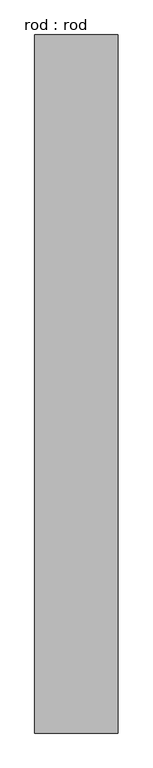
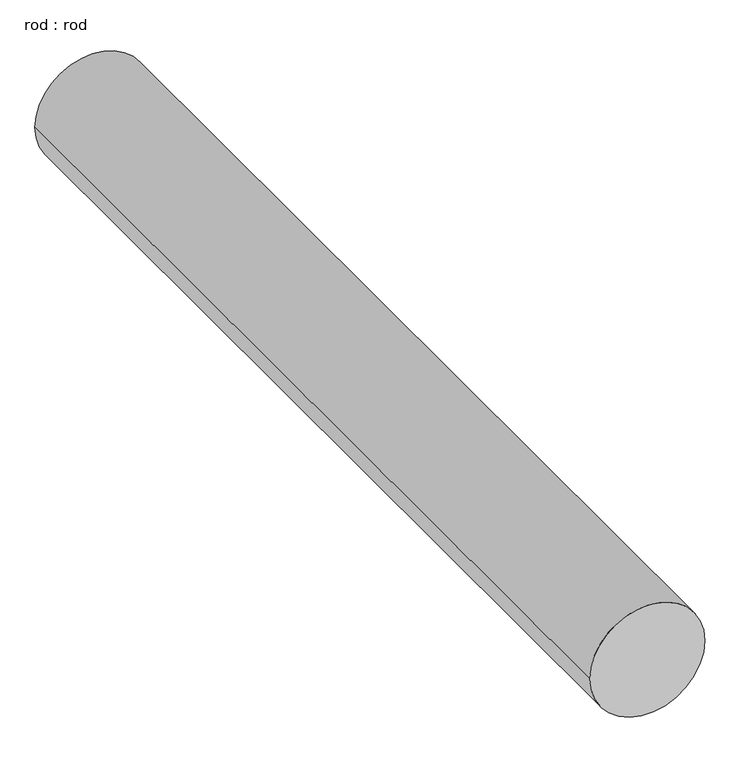
"""IFC4 building model written with IfcOpenShell, lengths in millimetres: proxy geometry, rod : rod."""

import ifcopenshell
import ifcopenshell.guid

model = None  # the IFC model being written
_history = None  # IfcOwnerHistory: only IFC2X3 demands one
_inside = {}  # id of a spatial element -> (the spatial element, [elements in it])
_under = {}  # id of a project, library or spatial element -> (it, [spatial elements below it])
_declared = {}  # id of a project -> (the project, [libraries it declares])
_typed = {}  # id of a type object -> (the type object, [elements of that type])
_made_of = {}  # id of a material, layer set ... -> (it, [elements and type objects made of it])


def new_model(schema):
    """Start an empty IFC model of exactly this schema.

    Asked for "IFC4X3", IfcOpenShell would pick the latest addendum, in which some entities
    have other attributes; the version numbers below select the first issue.
    IFC2X3 requires an IfcOwnerHistory on every rooted entity: one is made here for all.
    """
    global model, _history
    if schema == "IFC4X3":
        model = ifcopenshell.file(schema_version=(4, 3, 0, 0))
    else:
        model = ifcopenshell.file(schema=schema)
    _inside.clear()
    _under.clear()
    _declared.clear()
    _typed.clear()
    _made_of.clear()
    _history = None
    if model.schema == "IFC2X3":
        org = make("IfcOrganization", Name="unknown")
        user = make(
            "IfcPersonAndOrganization",
            ThePerson=make("IfcPerson", FamilyName="unknown"),
            TheOrganization=org,
        )
        app = make(
            "IfcApplication",
            ApplicationDeveloper=org,
            Version="unknown",
            ApplicationFullName="unknown",
            ApplicationIdentifier="unknown",
        )
        _history = make(
            "IfcOwnerHistory",
            OwningUser=user,
            OwningApplication=app,
            ChangeAction="ADDED",
            CreationDate=0,
        )
    return model


def make(cls, **values):
    """One entity of the class cls with the attributes given. An attribute that is None is left unset."""
    return model.create_entity(
        cls, **{name: value for name, value in values.items() if value is not None}
    )


def rooted(cls, **values):
    """An entity with a GlobalId (a new one), such as an element, a storey or a relation."""
    return make(cls, GlobalId=ifcopenshell.guid.new(), OwnerHistory=_history, **values)


def si_unit(unit_type, name, prefix=None):
    """IfcSIUnit, for example si_unit("LENGTHUNIT", "METRE", prefix="MILLI")."""
    return make("IfcSIUnit", UnitType=unit_type, Prefix=prefix, Name=name)


def assignment(units):
    """IfcUnitAssignment: the units of a project."""
    return None if units is None else make("IfcUnitAssignment", Units=units)


def point(xyz):
    """IfcCartesianPoint."""
    return None if xyz is None else make("IfcCartesianPoint", Coordinates=xyz)


def direction(xyz):
    """IfcDirection."""
    return None if xyz is None else make("IfcDirection", DirectionRatios=xyz)


def frame(location, z_axis=None, x_axis=None):
    """IfcAxis2Placement3D, a coordinate frame: its origin and axes. An axis left out is left unset."""
    return make(
        "IfcAxis2Placement3D",
        Location=point(location),
        Axis=direction(z_axis),
        RefDirection=direction(x_axis),
    )


def frame_2d(location, x_axis=None):
    """IfcAxis2Placement2D, a coordinate frame in the plane: its origin and x axis."""
    return make(
        "IfcAxis2Placement2D", Location=point(location), RefDirection=direction(x_axis)
    )


def origin():
    """The frame at (0, 0, 0) with its axes left unset."""
    return frame((0.0, 0.0, 0.0))


def place(relative_to, where):
    """IfcLocalPlacement: puts the frame where relative to a parent placement (None: the world)."""
    return make(
        "IfcLocalPlacement", PlacementRelTo=relative_to, RelativePlacement=where
    )


def context(
    kind, dimensions, precision=None, world=None, true_north=None, identifier=None
):
    """IfcGeometricRepresentationContext, for example the 3D "Model" context."""
    return make(
        "IfcGeometricRepresentationContext",
        ContextIdentifier=identifier,
        ContextType=kind,
        CoordinateSpaceDimension=dimensions,
        Precision=precision,
        WorldCoordinateSystem=world,
        TrueNorth=true_north,
    )


def project(units=None, contexts=None):
    """IfcProject with its units and contexts."""
    return rooted(
        "IfcProject",
        Name="project",
        RepresentationContexts=contexts,
        UnitsInContext=assignment(units),
    )


def spatial(cls, under=None, at=None, **own):
    """A site, building, storey or space (cls), placed at a placement, below another one or the project."""
    s = rooted(cls, ObjectPlacement=at, **own)
    if under is not None:
        _under.setdefault(under.id(), (under, []))[1].append(s)
    return s


def circle_curve(where, radius):
    """IfcCircle in the frame where."""
    return make("IfcCircle", Position=where, Radius=radius)


def trimmed(basis, trim1, trim2, sense, master):
    """IfcTrimmedCurve: the piece of a basis curve between two trims."""
    return make(
        "IfcTrimmedCurve",
        BasisCurve=basis,
        Trim1=trim1,
        Trim2=trim2,
        SenseAgreement=sense,
        MasterRepresentation=master,
    )


def segment(curve, same_sense, transition):
    """IfcCompositeCurveSegment."""
    return make(
        "IfcCompositeCurveSegment",
        Transition=transition,
        SameSense=same_sense,
        ParentCurve=curve,
    )


def composite_curve(segments, self_intersect=None):
    """IfcCompositeCurve: segments joined end to end."""
    return make("IfcCompositeCurve", Segments=segments, SelfIntersect=self_intersect)


def outline(outer, holes=None, kind="AREA"):
    """IfcArbitraryClosedProfileDef: a profile drawn as a closed curve; with holes, ...WithVoids."""
    if holes is None:
        return make("IfcArbitraryClosedProfileDef", ProfileType=kind, OuterCurve=outer)
    return make(
        "IfcArbitraryProfileDefWithVoids",
        ProfileType=kind,
        OuterCurve=outer,
        InnerCurves=holes,
    )


def extrude(swept, where, along, depth):
    """IfcExtrudedAreaSolid: the profile swept, set in the frame where, extruded along a direction by depth."""
    return make(
        "IfcExtrudedAreaSolid",
        SweptArea=swept,
        Position=where,
        ExtrudedDirection=direction(along),
        Depth=depth,
    )


def shape(context_of_items, identifier, shape_type, items):
    """IfcShapeRepresentation: the items that make up one representation, for example the "Body"."""
    return make(
        "IfcShapeRepresentation",
        ContextOfItems=context_of_items,
        RepresentationIdentifier=identifier,
        RepresentationType=shape_type,
        Items=items,
    )


def source(mapping_origin, context_of_items, identifier, shape_type, items):
    """IfcRepresentationMap: a shape defined once, which mapped items show again and again."""
    return make(
        "IfcRepresentationMap",
        MappingOrigin=mapping_origin,
        MappedRepresentation=shape(context_of_items, identifier, shape_type, items),
    )


def transform(
    local_origin,
    x_axis=None,
    y_axis=None,
    z_axis=None,
    scale=None,
    scale2=None,
    scale3=None,
    uniform=True,
):
    """IfcCartesianTransformationOperator3D, or its non-uniform kind. x_axis, y_axis, z_axis: its Axis1, 2, 3."""
    if uniform:
        return make(
            "IfcCartesianTransformationOperator3D",
            Axis1=direction(x_axis),
            Axis2=direction(y_axis),
            LocalOrigin=point(local_origin),
            Scale=scale,
            Axis3=direction(z_axis),
        )
    return make(
        "IfcCartesianTransformationOperator3DnonUniform",
        Axis1=direction(x_axis),
        Axis2=direction(y_axis),
        LocalOrigin=point(local_origin),
        Scale=scale,
        Axis3=direction(z_axis),
        Scale2=scale2,
        Scale3=scale3,
    )


def mapped(mapping_source, mapping_target):
    """IfcMappedItem: shows the shape of a source again, moved by a transform."""
    return make(
        "IfcMappedItem", MappingSource=mapping_source, MappingTarget=mapping_target
    )


def made_of(thing, what):
    """Note that an element or type object is made of a material, layer set ...; save() writes the relation."""
    if what is not None:
        _made_of.setdefault(what.id(), (what, []))[1].append(thing)
    return thing


def element(
    cls,
    number,
    at=None,
    inside=None,
    cuts=None,
    type_object=None,
    material=None,
    context=None,
    identifier="Body",
    shape_type=None,
    held_by="IfcProductDefinitionShape",
    body=None,
    shapes=None,
    **own,
):
    """One element of the class cls, such as IfcWall. Its Tag is "e" and its number.

    at: its placement. inside: the storey or other place that contains it. cuts: it is an
    opening in that element (IfcRelVoidsElement). A single representation is given by context,
    identifier, shape_type and body (its items); several are given by shapes. held_by: the class
    of the entity that holds the representations. save() writes the other relations.
    """
    e = rooted(cls, Tag="e%d" % number, ObjectPlacement=at, **own)
    if body is not None:
        shapes = [shape(context, identifier, shape_type, body)]
    if shapes is not None:
        e.Representation = make(held_by, Representations=shapes)
    if inside is not None:
        _inside.setdefault(inside.id(), (inside, []))[1].append(e)
    if cuts is not None:
        rooted(
            "IfcRelVoidsElement", RelatingBuildingElement=cuts, RelatedOpeningElement=e
        )
    if type_object is not None:
        _typed.setdefault(type_object.id(), (type_object, []))[1].append(e)
    return made_of(e, material)


def aggregate(whole, parts):
    """IfcRelAggregates: a whole, such as a stair, and the parts it consists of."""
    return rooted("IfcRelAggregates", RelatingObject=whole, RelatedObjects=parts)


def save(model, path):
    """Write the relations noted so far, then the file.

    IfcRelAggregates (storeys below a building ...), IfcRelContainedInSpatialStructure (elements
    in a storey), IfcRelDefinesByType, IfcRelAssociatesMaterial and IfcRelDeclares: one each for
    every whole, place, type object, material and project.
    """
    for whole, parts in _under.values():
        aggregate(whole, parts)
    for where, things in _inside.values():
        rooted(
            "IfcRelContainedInSpatialStructure",
            RelatedElements=things,
            RelatingStructure=where,
        )
    for kind, things in _typed.values():
        rooted("IfcRelDefinesByType", RelatedObjects=things, RelatingType=kind)
    for what, things in _made_of.values():
        rooted("IfcRelAssociatesMaterial", RelatedObjects=things, RelatingMaterial=what)
    for by, libraries in _declared.values():
        rooted("IfcRelDeclares", RelatingContext=by, RelatedDefinitions=libraries)
    model.write(path)


def rod_rod_bf858b28(model_context):
    return source(origin(), model_context, "Body", "SweptSolid", [
        extrude(outline(composite_curve([segment(trimmed(circle_curve(frame_2d((0.0108462, 0.0)), 200.0), [point((0.0108462, 200.0))], [point((0.0108462, -200.0))], False, "CARTESIAN"), True, "CONTINUOUS"), segment(trimmed(circle_curve(frame_2d((0.0108462, 0.0)), 200.0), [point((0.0108462, -200.0))], [point((0.0108462, 200.0))], False, "CARTESIAN"), True, "CONTINUOUS")], self_intersect=False)), frame((0.0, 2421.3000439, 0.0), z_axis=(0.0, 1.0, 0.0), x_axis=(0.0, 0.0, 1.0)), (0.0, 0.0, 1.0), 3342.8571429),
    ])


if __name__ == "__main__":
    model = new_model("IFC4")
    model_context = context("Model", 3, world=origin())
    ifc_project = project(units=[si_unit("LENGTHUNIT", "METRE", prefix="MILLI")], contexts=[model_context])
    site = spatial("IfcSite", under=ifc_project)
    building = spatial("IfcBuilding", under=site)
    placement = place(None, origin())
    rod_rod_shape = rod_rod_bf858b28(model_context)
    element("IfcBuildingElementProxy", 1, Name="rod : rod", ObjectType="rod : rod", at=placement, inside=building, context=model_context, shape_type="MappedRepresentation", body=[
        mapped(rod_rod_shape, transform((0.0, 0.0, 0.0), x_axis=(1.0, 0.0, 0.0), y_axis=(0.0, 1.0, 0.0), z_axis=(0.0, 0.0, 1.0))),
    ])
    save(model, "model.ifc")

# Revit data of these elements
# Type "rod : rod"
#   Default Elevation = 0
